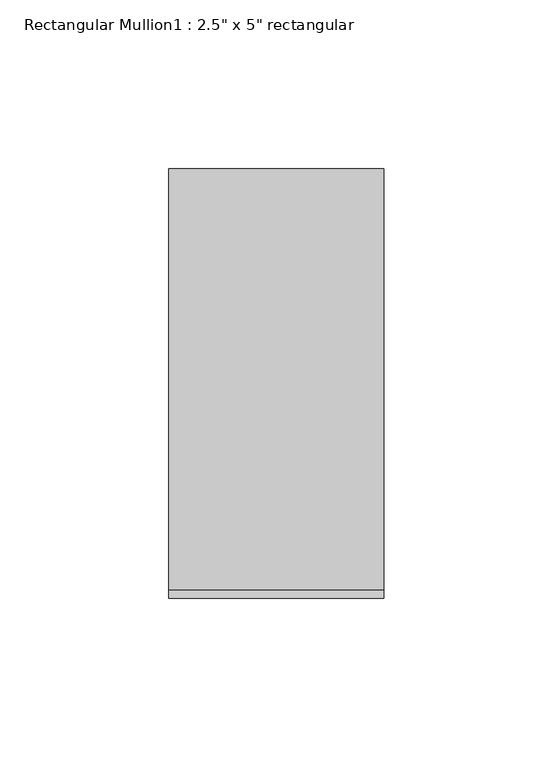
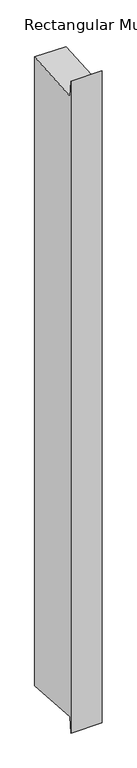
"""IFC4 building model written with IfcOpenShell, lengths in millimetres: member geometry."""

from ifc_helpers import new_model, si_unit, frame, origin, place, context, project, spatial, polyline, outline, extrude, source, transform, mapped, element, save


def member_233ab79f(model_context):
    return source(origin(), model_context, "Body", "SweptSolid", [
        extrude(outline(polyline([(-63.5, 29.4471051), (-61.0333155, -4.5163328), (63.5, 4.5282284), (63.5, -1343.9489353), (-61.0333155, -1334.904374), (-63.5, -1368.8678119), (-63.5, 29.4471051)])), frame((-63.5, 0.0, 0.0), z_axis=(1.0, 0.0, 0.0), x_axis=(0.0, 1.0, 0.0)), (0.0, 0.0, 1.0), 63.5),
    ])


if __name__ == "__main__":
    model = new_model("IFC4")
    model_context = context("Model", 3, world=origin())
    ifc_project = project(units=[si_unit("LENGTHUNIT", "METRE", prefix="MILLI")], contexts=[model_context])
    site = spatial("IfcSite", under=ifc_project)
    building = spatial("IfcBuilding", under=site)
    placement = place(None, origin())
    member_shape = member_233ab79f(model_context)
    element("IfcMember", 1, ObjectType="Rectangular Mullion1 : 2.5\" x 5\" rectangular", at=placement, inside=building, context=model_context, shape_type="MappedRepresentation", body=[
        mapped(member_shape, transform((0.0, 0.0, 0.0), x_axis=(1.0, 0.0, 0.0), y_axis=(0.0, 1.0, 0.0), z_axis=(0.0, 0.0, 1.0))),
    ])
    save(model, "model.ifc")

# Revit data of these elements
# Type "Rectangular Mullion1 : 2.5\" x 5\" rectangular"
#   built-in parameter 1007304 = 0.416667 (stored number, unit not read)
#   built-in parameter 1007301 = 0.104167 (stored number, unit not read)
#   built-in parameter 1007300 = 0.104167 (stored number, unit not read)
# Element 1 (IfcMember, "Rectangular Mullion1 : 2.5\" x 5\" rectangular")
#   Materials on its faces: "support-frame"
# Materials
#   "support-frame": class "Unassigned", colour RGB 233 233 233, transparency 0, Cost = 0
